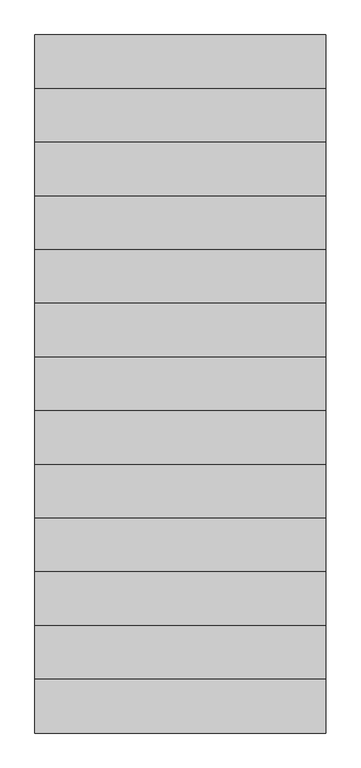
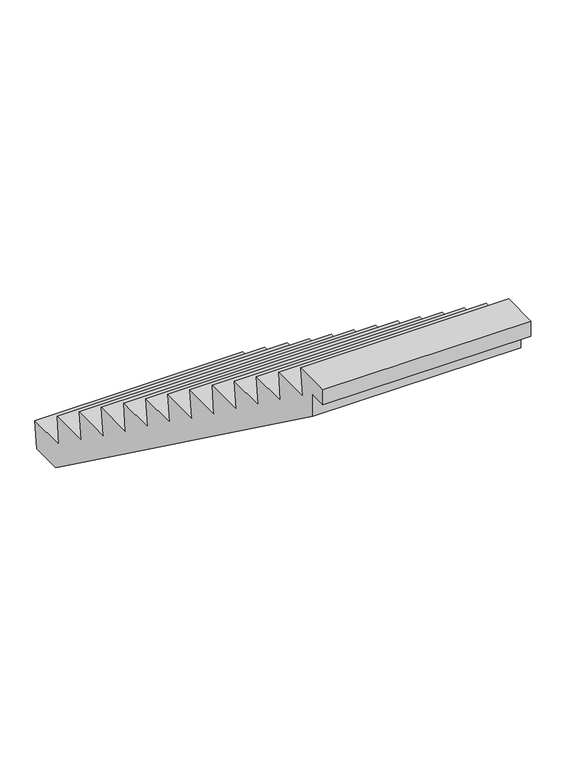
"""IFC4 building model written with IfcOpenShell, lengths in millimetres: stair geometry, NLRS_24_GM_LB_rechte steektrap prefab-AV_gen_rsf : prefab trap_gen__aant=12 b=1200 a=220 o=172.7 zonder bomen."""

from ifc_helpers import new_model, si_unit, frame, origin, place, context, project, spatial, polyline, outline, extrude, source, transform, mapped, element, save


def stair_37fa75c9(model_context):
    return source(origin(), model_context, "Body", "SweptSolid", [
        extrude(outline(polyline([(-2880.0, 2270.0), (-2900.0, 2095.3846154), (-2640.0, 2095.3846154), (-2660.0, 1920.7692308), (-2400.0, 1920.7692308), (-2420.0, 1746.1538462), (-2160.0, 1746.1538462), (-2180.0, 1571.5384615), (-1920.0, 1571.5384615), (-1940.0, 1396.9230769), (-1680.0, 1396.9230769), (-1700.0, 1222.3076923), (-1440.0, 1222.3076923), (-1460.0, 1047.6923077), (-1200.0, 1047.6923077), (-1220.0, 873.0769231), (-960.0, 873.0769231), (-980.0, 698.4615385), (-720.0, 698.4615385), (-740.0, 523.8461538), (-480.0, 523.8461538), (-500.0, 349.2307692), (-240.0, 349.2307692), (-260.0, 174.6153846), (0.0, 174.6153846), (-20.0, 0.0), (-223.9686206, 0.0), (-3010.0, 2027.0164203), (-3010.0, 2170.0), (-3120.0, 2170.0), (-3120.0, 2270.0), (-2880.0, 2270.0)])), frame((-650.0, 0.0, 0.0), z_axis=(1.0, 0.0, 0.0), x_axis=(0.0, 1.0, 0.0)), (0.0, 0.0, 1.0), 1300.0),
    ])


if __name__ == "__main__":
    model = new_model("IFC4")
    model_context = context("Model", 3, world=origin())
    ifc_project = project(units=[si_unit("LENGTHUNIT", "METRE", prefix="MILLI")], contexts=[model_context])
    site = spatial("IfcSite", under=ifc_project)
    building = spatial("IfcBuilding", under=site)
    placement = place(None, origin())
    stair_shape = stair_37fa75c9(model_context)
    element("IfcStair", 1, ObjectType="NLRS_24_GM_LB_rechte steektrap prefab-AV_gen_rsf : prefab trap_gen__aant=12 b=1200 a=220 o=172.7 zonder bomen", at=placement, inside=building, context=model_context, shape_type="MappedRepresentation", body=[
        mapped(stair_shape, transform((0.0, 0.0, 0.0), x_axis=(1.0, 0.0, 0.0), y_axis=(0.0, 1.0, 0.0), z_axis=(0.0, 0.0, 1.0))),
    ])
    save(model, "model.ifc")

# Revit data of these elements
# Type "NLRS_24_GM_LB_rechte steektrap prefab-AV_gen_rsf : prefab trap_gen__aant=12 b=1200 a=220 o=172.7 zonder bomen"
#   IfcExportAs = "IfcStair"
#   Type Comments = " "
#   Model = " "
#   Manufacturer = " "
#   Keynote = " "
#   Description = "rechte steektrap prefab\r\naant=11 b=1200 a=220 o=181,8\r\nzonder bomen"
#   Assembly Code = "24.11"
#   Aantrede onder = 240 mm
#   Width = 1300 mm
#   Wel diepte = 20 mm
#   Trapboom breedte = 0 mm
#   Thickness = 120 mm
#   Optrede onderste trede = 150 mm
#   NLRS_C_lengte = 2880 mm
#   Length = 3360 mm
#   Hoogte oplegnok onder = 100 mm
#   Hoogte oplegnok boven = 100 mm
#   Height = 2270 mm
#   Breedte oplegnok boven = 110 mm
#   BottomCalc = 150 mm
#   Actual Tread Depth = 240 mm
#   Actual Riser Height = 174.615 mm
#   Actual Number of Tread = 12
#   Actual Number of Risers = 13
#   Aantrede boven = 240 mm
#   Aantal treden max dertig = 13
#   Trapboom = no
#   Oplegnok onder = no
#   NLRS_C_materiaal = NLRS_f2_beton prefab_gen_rsf
#   Default Elevation = 0
# Element 1 (IfcStair, "NLRS_24_GM_LB_rechte steektrap prefab-AV_gen_rsf : prefab trap_gen__aant=12 b=1200 a=220 o=172.7 zonder bomen")
#   Materials on its faces: "NLRS_f2_beton prefab_gen_rsf"
# Materials
#   "NLRS_f2_beton prefab_gen_rsf": class "F - Niet gebakken kunststeen", colour RGB 129 133 118, transparency 0, Keynote = "f2", Manufacturer = "Revit Standards Foundation", URL = "www.revitstandards.org", Description = "beton prefab", Cost = 0
